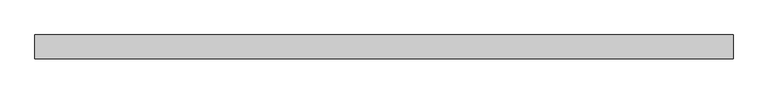
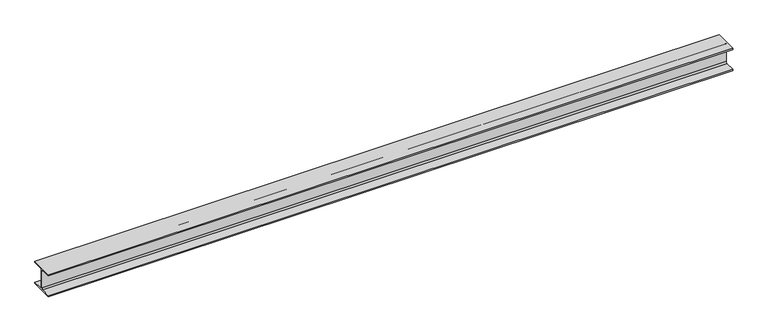
"""IFC4 building model written with IfcOpenShell, lengths in millimetres: beam geometry, 0912_Steel Framing_H-KSD3502 : H_SB_ASB_H-200x200x8x12."""

import ifcopenshell
import ifcopenshell.guid

model = None  # the IFC model being written
_history = None  # IfcOwnerHistory: only IFC2X3 demands one
_inside = {}  # id of a spatial element -> (the spatial element, [elements in it])
_under = {}  # id of a project, library or spatial element -> (it, [spatial elements below it])
_declared = {}  # id of a project -> (the project, [libraries it declares])
_typed = {}  # id of a type object -> (the type object, [elements of that type])
_made_of = {}  # id of a material, layer set ... -> (it, [elements and type objects made of it])


def new_model(schema):
    """Start an empty IFC model of exactly this schema.

    Asked for "IFC4X3", IfcOpenShell would pick the latest addendum, in which some entities
    have other attributes; the version numbers below select the first issue.
    IFC2X3 requires an IfcOwnerHistory on every rooted entity: one is made here for all.
    """
    global model, _history
    if schema == "IFC4X3":
        model = ifcopenshell.file(schema_version=(4, 3, 0, 0))
    else:
        model = ifcopenshell.file(schema=schema)
    _inside.clear()
    _under.clear()
    _declared.clear()
    _typed.clear()
    _made_of.clear()
    _history = None
    if model.schema == "IFC2X3":
        org = make("IfcOrganization", Name="unknown")
        user = make(
            "IfcPersonAndOrganization",
            ThePerson=make("IfcPerson", FamilyName="unknown"),
            TheOrganization=org,
        )
        app = make(
            "IfcApplication",
            ApplicationDeveloper=org,
            Version="unknown",
            ApplicationFullName="unknown",
            ApplicationIdentifier="unknown",
        )
        _history = make(
            "IfcOwnerHistory",
            OwningUser=user,
            OwningApplication=app,
            ChangeAction="ADDED",
            CreationDate=0,
        )
    return model


def make(cls, **values):
    """One entity of the class cls with the attributes given. An attribute that is None is left unset."""
    return model.create_entity(
        cls, **{name: value for name, value in values.items() if value is not None}
    )


def rooted(cls, **values):
    """An entity with a GlobalId (a new one), such as an element, a storey or a relation."""
    return make(cls, GlobalId=ifcopenshell.guid.new(), OwnerHistory=_history, **values)


def si_unit(unit_type, name, prefix=None):
    """IfcSIUnit, for example si_unit("LENGTHUNIT", "METRE", prefix="MILLI")."""
    return make("IfcSIUnit", UnitType=unit_type, Prefix=prefix, Name=name)


def assignment(units):
    """IfcUnitAssignment: the units of a project."""
    return None if units is None else make("IfcUnitAssignment", Units=units)


def point(xyz):
    """IfcCartesianPoint."""
    return None if xyz is None else make("IfcCartesianPoint", Coordinates=xyz)


def direction(xyz):
    """IfcDirection."""
    return None if xyz is None else make("IfcDirection", DirectionRatios=xyz)


def frame(location, z_axis=None, x_axis=None):
    """IfcAxis2Placement3D, a coordinate frame: its origin and axes. An axis left out is left unset."""
    return make(
        "IfcAxis2Placement3D",
        Location=point(location),
        Axis=direction(z_axis),
        RefDirection=direction(x_axis),
    )


def frame_2d(location, x_axis=None):
    """IfcAxis2Placement2D, a coordinate frame in the plane: its origin and x axis."""
    return make(
        "IfcAxis2Placement2D", Location=point(location), RefDirection=direction(x_axis)
    )


def origin():
    """The frame at (0, 0, 0) with its axes left unset."""
    return frame((0.0, 0.0, 0.0))


def place(relative_to, where):
    """IfcLocalPlacement: puts the frame where relative to a parent placement (None: the world)."""
    return make(
        "IfcLocalPlacement", PlacementRelTo=relative_to, RelativePlacement=where
    )


def context(
    kind, dimensions, precision=None, world=None, true_north=None, identifier=None
):
    """IfcGeometricRepresentationContext, for example the 3D "Model" context."""
    return make(
        "IfcGeometricRepresentationContext",
        ContextIdentifier=identifier,
        ContextType=kind,
        CoordinateSpaceDimension=dimensions,
        Precision=precision,
        WorldCoordinateSystem=world,
        TrueNorth=true_north,
    )


def project(units=None, contexts=None):
    """IfcProject with its units and contexts."""
    return rooted(
        "IfcProject",
        Name="project",
        RepresentationContexts=contexts,
        UnitsInContext=assignment(units),
    )


def spatial(cls, under=None, at=None, **own):
    """A site, building, storey or space (cls), placed at a placement, below another one or the project."""
    s = rooted(cls, ObjectPlacement=at, **own)
    if under is not None:
        _under.setdefault(under.id(), (under, []))[1].append(s)
    return s


def polyline(points):
    """IfcPolyline through the points."""
    return make("IfcPolyline", Points=[point(p) for p in points])


def circle_curve(where, radius):
    """IfcCircle in the frame where."""
    return make("IfcCircle", Position=where, Radius=radius)


def trimmed(basis, trim1, trim2, sense, master):
    """IfcTrimmedCurve: the piece of a basis curve between two trims."""
    return make(
        "IfcTrimmedCurve",
        BasisCurve=basis,
        Trim1=trim1,
        Trim2=trim2,
        SenseAgreement=sense,
        MasterRepresentation=master,
    )


def segment(curve, same_sense, transition):
    """IfcCompositeCurveSegment."""
    return make(
        "IfcCompositeCurveSegment",
        Transition=transition,
        SameSense=same_sense,
        ParentCurve=curve,
    )


def composite_curve(segments, self_intersect=None):
    """IfcCompositeCurve: segments joined end to end."""
    return make("IfcCompositeCurve", Segments=segments, SelfIntersect=self_intersect)


def outline(outer, holes=None, kind="AREA"):
    """IfcArbitraryClosedProfileDef: a profile drawn as a closed curve; with holes, ...WithVoids."""
    if holes is None:
        return make("IfcArbitraryClosedProfileDef", ProfileType=kind, OuterCurve=outer)
    return make(
        "IfcArbitraryProfileDefWithVoids",
        ProfileType=kind,
        OuterCurve=outer,
        InnerCurves=holes,
    )


def extrude(swept, where, along, depth):
    """IfcExtrudedAreaSolid: the profile swept, set in the frame where, extruded along a direction by depth."""
    return make(
        "IfcExtrudedAreaSolid",
        SweptArea=swept,
        Position=where,
        ExtrudedDirection=direction(along),
        Depth=depth,
    )


def shape(context_of_items, identifier, shape_type, items):
    """IfcShapeRepresentation: the items that make up one representation, for example the "Body"."""
    return make(
        "IfcShapeRepresentation",
        ContextOfItems=context_of_items,
        RepresentationIdentifier=identifier,
        RepresentationType=shape_type,
        Items=items,
    )


def source(mapping_origin, context_of_items, identifier, shape_type, items):
    """IfcRepresentationMap: a shape defined once, which mapped items show again and again."""
    return make(
        "IfcRepresentationMap",
        MappingOrigin=mapping_origin,
        MappedRepresentation=shape(context_of_items, identifier, shape_type, items),
    )


def transform(
    local_origin,
    x_axis=None,
    y_axis=None,
    z_axis=None,
    scale=None,
    scale2=None,
    scale3=None,
    uniform=True,
):
    """IfcCartesianTransformationOperator3D, or its non-uniform kind. x_axis, y_axis, z_axis: its Axis1, 2, 3."""
    if uniform:
        return make(
            "IfcCartesianTransformationOperator3D",
            Axis1=direction(x_axis),
            Axis2=direction(y_axis),
            LocalOrigin=point(local_origin),
            Scale=scale,
            Axis3=direction(z_axis),
        )
    return make(
        "IfcCartesianTransformationOperator3DnonUniform",
        Axis1=direction(x_axis),
        Axis2=direction(y_axis),
        LocalOrigin=point(local_origin),
        Scale=scale,
        Axis3=direction(z_axis),
        Scale2=scale2,
        Scale3=scale3,
    )


def mapped(mapping_source, mapping_target):
    """IfcMappedItem: shows the shape of a source again, moved by a transform."""
    return make(
        "IfcMappedItem", MappingSource=mapping_source, MappingTarget=mapping_target
    )


def made_of(thing, what):
    """Note that an element or type object is made of a material, layer set ...; save() writes the relation."""
    if what is not None:
        _made_of.setdefault(what.id(), (what, []))[1].append(thing)
    return thing


def element(
    cls,
    number,
    at=None,
    inside=None,
    cuts=None,
    type_object=None,
    material=None,
    context=None,
    identifier="Body",
    shape_type=None,
    held_by="IfcProductDefinitionShape",
    body=None,
    shapes=None,
    **own,
):
    """One element of the class cls, such as IfcWall. Its Tag is "e" and its number.

    at: its placement. inside: the storey or other place that contains it. cuts: it is an
    opening in that element (IfcRelVoidsElement). A single representation is given by context,
    identifier, shape_type and body (its items); several are given by shapes. held_by: the class
    of the entity that holds the representations. save() writes the other relations.
    """
    e = rooted(cls, Tag="e%d" % number, ObjectPlacement=at, **own)
    if body is not None:
        shapes = [shape(context, identifier, shape_type, body)]
    if shapes is not None:
        e.Representation = make(held_by, Representations=shapes)
    if inside is not None:
        _inside.setdefault(inside.id(), (inside, []))[1].append(e)
    if cuts is not None:
        rooted(
            "IfcRelVoidsElement", RelatingBuildingElement=cuts, RelatedOpeningElement=e
        )
    if type_object is not None:
        _typed.setdefault(type_object.id(), (type_object, []))[1].append(e)
    return made_of(e, material)


def aggregate(whole, parts):
    """IfcRelAggregates: a whole, such as a stair, and the parts it consists of."""
    return rooted("IfcRelAggregates", RelatingObject=whole, RelatedObjects=parts)


def save(model, path):
    """Write the relations noted so far, then the file.

    IfcRelAggregates (storeys below a building ...), IfcRelContainedInSpatialStructure (elements
    in a storey), IfcRelDefinesByType, IfcRelAssociatesMaterial and IfcRelDeclares: one each for
    every whole, place, type object, material and project.
    """
    for whole, parts in _under.values():
        aggregate(whole, parts)
    for where, things in _inside.values():
        rooted(
            "IfcRelContainedInSpatialStructure",
            RelatedElements=things,
            RelatingStructure=where,
        )
    for kind, things in _typed.values():
        rooted("IfcRelDefinesByType", RelatedObjects=things, RelatingType=kind)
    for what, things in _made_of.values():
        rooted("IfcRelAssociatesMaterial", RelatedObjects=things, RelatingMaterial=what)
    for by, libraries in _declared.values():
        rooted("IfcRelDeclares", RelatingContext=by, RelatedDefinitions=libraries)
    model.write(path)


def beam_c011c040(model_context):
    return source(origin(), model_context, "Body", "SweptSolid", [
        extrude(outline(composite_curve([segment(polyline([(100.0, -88.0), (100.0, -100.0), (-100.0, -100.0), (-100.0, -88.0), (-17.0, -88.0)]), True, "CONTINUOUS"), segment(trimmed(circle_curve(frame_2d((-17.0, -75.0)), 13.0), [point((-17.0, -88.0))], [point((-4.0, -75.0))], True, "CARTESIAN"), True, "CONTINUOUS"), segment(polyline([(-4.0, -75.0), (-4.0, 75.0)]), True, "CONTINUOUS"), segment(trimmed(circle_curve(frame_2d((-17.0, 75.0)), 13.0), [point((-4.0, 75.0))], [point((-17.0, 88.0))], True, "CARTESIAN"), True, "CONTINUOUS"), segment(polyline([(-17.0, 88.0), (-100.0, 88.0), (-100.0, 100.0), (100.0, 100.0), (100.0, 88.0), (17.0, 88.0)]), True, "CONTINUOUS"), segment(trimmed(circle_curve(frame_2d((17.0, 75.0)), 13.0), [point((17.0, 88.0))], [point((4.0, 75.0))], True, "CARTESIAN"), True, "CONTINUOUS"), segment(polyline([(4.0, 75.0), (4.0, -75.0)]), True, "CONTINUOUS"), segment(trimmed(circle_curve(frame_2d((17.0, -75.0)), 13.0), [point((4.0, -75.0))], [point((17.0, -88.0))], True, "CARTESIAN"), True, "CONTINUOUS"), segment(polyline([(17.0, -88.0), (100.0, -88.0)]), True, "CONTINUOUS")], self_intersect=False)), frame((-3108.0679819, 0.0, 0.0), z_axis=(1.0, 0.0, 0.0), x_axis=(0.0, 1.0, 0.0)), (0.0, 0.0, 1.0), 5816.9163649),
    ])


if __name__ == "__main__":
    model = new_model("IFC4")
    model_context = context("Model", 3, world=origin())
    ifc_project = project(units=[si_unit("LENGTHUNIT", "METRE", prefix="MILLI")], contexts=[model_context])
    site = spatial("IfcSite", under=ifc_project)
    building = spatial("IfcBuilding", under=site)
    placement = place(None, origin())
    beam_shape = beam_c011c040(model_context)
    element("IfcBeam", 1, ObjectType="0912_Steel Framing_H-KSD3502 : H_SB_ASB_H-200x200x8x12", at=placement, inside=building, context=model_context, shape_type="MappedRepresentation", body=[
        mapped(beam_shape, transform((0.0, 0.0, 0.0), x_axis=(1.0, 0.0, 0.0), y_axis=(0.0, 1.0, 0.0), z_axis=(0.0, 0.0, 1.0))),
    ])
    save(model, "model.ifc")

# Revit data of these elements
# Type "0912_Steel Framing_H-KSD3502 : H_SB_ASB_H-200x200x8x12"
#   H_WM Code_1 = "S01AA002-00001 | Main Steel Structure Fabrication Work | Shelter/Building | Medium Steel - Standard (90KG/M>Weight≥30KG/M) | Material: (   )"
#   H_WM Code_2 = "S03AA028-00001 | Main Steel Structure Erection Work | Shelter/Building | Medium Steel (90KG/M>Weight≥30KG/M) | Material: (   )"
#   H_WM Code_3 = "S01AA010-00001 | Main Steel Structure Fabrication Work | Shelter/Building | Steel Painting/Coating | for Non-Fireproofed Steel Surface, Surface Preparation, Primer, Second & Final Coat | Material: (   )"
#   H_Q'ty Cal Type Tag = "SB-Q2"
#   Width = 20.0 cm
#   Web Thickness = 0.8 cm
#   Web Fillet = 1.3 cm
#   Warping Constant = 141000.0 cm⁶
#   W = 0
#   Torsional Moment of Inertia = 26.2485 cm⁴
#   Section Area = 63.53 cm²
#   Plastic Modulus weak axis = 244.0 cm³
#   Plastic Modulus strong axis = 525.0 cm³
#   Perimeter = 1.16 m²/m
#   Nominal Weight = 49.90 kgf/m
#   Moment of Inertia weak axis = 1600.00 cm⁴
#   Moment of Inertia strong axis = 4720.00 cm⁴
#   Height = 20.0 cm
#   Flange Thickness = 1.2 cm
#   Elastic Modulus weak axis = 160.0 cm³
#   Elastic Modulus strong axis = 472.0 cm³
#   Centroid Vertical = 10.0 cm
#   Centroid Horizontal = 10.0 cm
#   Ix = 47200000
#   Length [instance default] = 1.5240 m
#   Zx = 525000
#   b = 0.2000 m
#   h = 0.2000 m
#   r = 0.0130 m
#   s = 0.0080 m
#   t = 0.0120 m
#   A = 0.006353 m²
#   Structural Material [instance default] = Steel, 45-345
#   Assembly Code = ""
# Element 1 (IfcBeam, "0912_Steel Framing_H-KSD3502 : H_SB_ASB_H-200x200x8x12")
#   Structural Material = none
# Materials
#   "Steel, 45-345": class "Metal", colour RGB 189 187 185, transparency 0, Description = "Steel 345 MPa", Cost = 0
